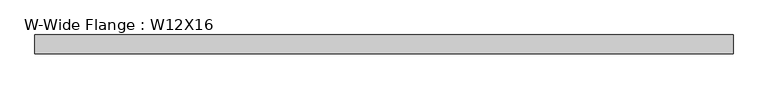
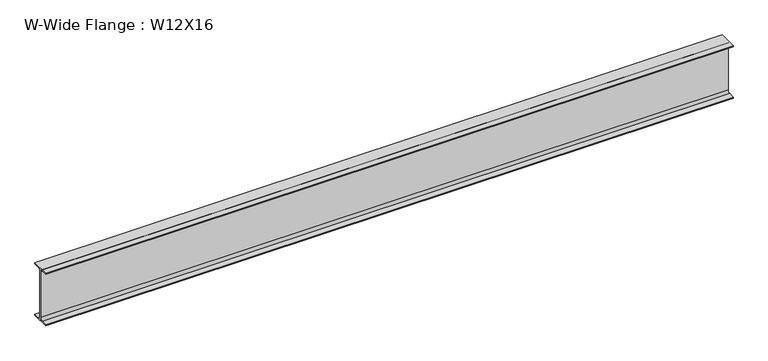
"""IFC4 building model written with IfcOpenShell, lengths in millimetres: beam geometry, W-Wide Flange : W12X16."""

from ifc_helpers import new_model, si_unit, point, frame, frame_2d, origin, place, context, project, spatial, polyline, circle_curve, trimmed, segment, composite_curve, outline, extrude, source, transform, mapped, element, save


def w_wide_flange_w12x16_bc225ebf(model_context):
    return source(origin(), model_context, "Body", "SweptSolid", [
        extrude(outline(composite_curve([segment(polyline([(50.673, -145.669), (50.673, -152.4), (-50.673, -152.4), (-50.673, -145.669), (-16.7005, -145.669)]), True, "CONTINUOUS"), segment(trimmed(circle_curve(frame_2d((-16.7005, -131.7625)), 13.9065), [point((-16.7005, -145.669))], [point((-2.794, -131.7625))], True, "CARTESIAN"), True, "CONTINUOUS"), segment(polyline([(-2.794, -131.7625), (-2.794, 131.7625)]), True, "CONTINUOUS"), segment(trimmed(circle_curve(frame_2d((-16.7005, 131.7625)), 13.9065), [point((-2.794, 131.7625))], [point((-16.7005, 145.669))], True, "CARTESIAN"), True, "CONTINUOUS"), segment(polyline([(-16.7005, 145.669), (-50.673, 145.669), (-50.673, 152.4), (50.673, 152.4), (50.673, 145.669), (16.7005, 145.669)]), True, "CONTINUOUS"), segment(trimmed(circle_curve(frame_2d((16.7005, 131.7625)), 13.9065), [point((16.7005, 145.669))], [point((2.794, 131.7625))], True, "CARTESIAN"), True, "CONTINUOUS"), segment(polyline([(2.794, 131.7625), (2.794, -131.7625)]), True, "CONTINUOUS"), segment(trimmed(circle_curve(frame_2d((16.7005, -131.7625)), 13.9065), [point((2.794, -131.7625))], [point((16.7005, -145.669))], True, "CARTESIAN"), True, "CONTINUOUS"), segment(polyline([(16.7005, -145.669), (50.673, -145.669)]), True, "CONTINUOUS")], self_intersect=False)), frame((-1892.3, 0.0, 0.0), z_axis=(1.0, 0.0, 0.0), x_axis=(0.0, 1.0, 0.0)), (0.0, 0.0, 1.0), 3764.407),
    ])


if __name__ == "__main__":
    model = new_model("IFC4")
    model_context = context("Model", 3, world=origin())
    ifc_project = project(units=[si_unit("LENGTHUNIT", "METRE", prefix="MILLI")], contexts=[model_context])
    site = spatial("IfcSite", under=ifc_project)
    building = spatial("IfcBuilding", under=site)
    placement = place(None, origin())
    w_wide_flange_w12x16_shape = w_wide_flange_w12x16_bc225ebf(model_context)
    element("IfcBeam", 1, ObjectType="W-Wide Flange : W12X16", at=placement, inside=building, context=model_context, shape_type="MappedRepresentation", body=[
        mapped(w_wide_flange_w12x16_shape, transform((0.0, 0.0, 0.0), x_axis=(1.0, 0.0, 0.0), y_axis=(0.0, 1.0, 0.0), z_axis=(0.0, 0.0, 1.0))),
    ])
    save(model, "model.ifc")

# Revit data of these elements
# Type "W-Wide Flange : W12X16"
#   Assembly Code = "B10"
#   W = 16
#   Length [instance default] = 5' - 0"
#   bf = 0' - 3.99"
#   d = 1' - 0"
#   k = 0' - 0 13/16"
#   k2 = 0' - 0.5475"
#   tf = 0' - 0.265"
#   tw = 0' - 0.22"
#   A = 0.0327083 SF
#   Structural Material [instance default] = Steel ASTM A992
# Element 1 (IfcBeam, "W-Wide Flange : W12X16")
#   Materials on its faces: "Steel ASTM A992"
# Materials
#   "Steel ASTM A992": class "Metal", colour RGB 199 199 199, transparency 0, Description = "Structural steel 50ksi", Cost = 0
